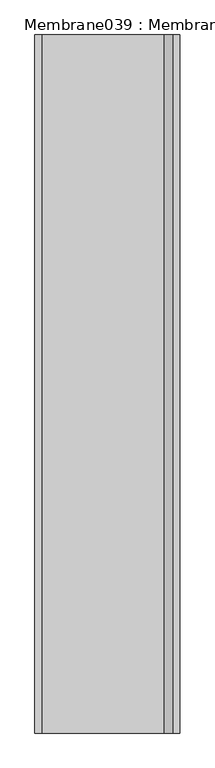
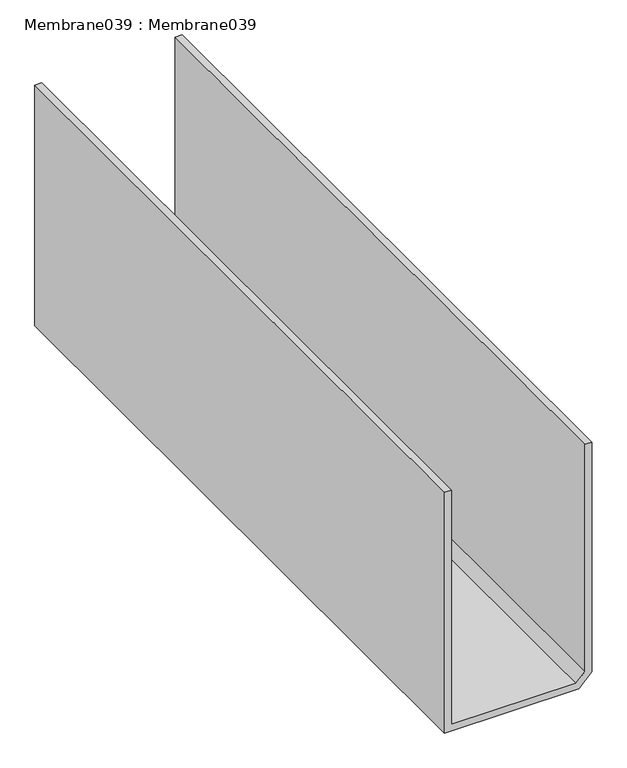
"""IFC4 building model written with IfcOpenShell, lengths in millimetres: proxy geometry, Membrane039 : Membrane039."""

from ifc_helpers import new_model, si_unit, frame, origin, place, context, project, spatial, polyline, outline, extrude, source, transform, mapped, element, save


def membrane039_membrane039_2a3038c1(model_context):
    return source(origin(), model_context, "Body", "SweptSolid", [
        extrude(outline(polyline([(33313.1445312, -9688.7902344), (32637.1367048, -9688.7902344), (32611.440625, -9714.2056282), (32611.440625, -10065.5505859), (33309.0146212, -10065.5505859), (33309.0146212, -10084.6005859), (32592.390625, -10084.6005859), (32592.390625, -9706.2535079), (32629.3071489, -9669.7402344), (33313.1445312, -9669.7402344), (33313.1445312, -9688.7902344)])), frame((0.0, 7982.1531721, 0.0), z_axis=(0.0, 1.0, 0.0), x_axis=(0.0, 0.0, 1.0)), (0.0, 0.0, 1.0), 2000.0),
    ])


if __name__ == "__main__":
    model = new_model("IFC4")
    model_context = context("Model", 3, world=origin())
    ifc_project = project(units=[si_unit("LENGTHUNIT", "METRE", prefix="MILLI")], contexts=[model_context])
    site = spatial("IfcSite", under=ifc_project)
    building = spatial("IfcBuilding", under=site)
    placement = place(None, origin())
    membrane039_membrane039_shape = membrane039_membrane039_2a3038c1(model_context)
    element("IfcBuildingElementProxy", 1, Name="Membrane039 : Membrane039", ObjectType="Membrane039 : Membrane039", at=placement, inside=building, context=model_context, shape_type="MappedRepresentation", body=[
        mapped(membrane039_membrane039_shape, transform((0.0, 0.0, 0.0), x_axis=(1.0, 0.0, 0.0), y_axis=(0.0, 1.0, 0.0), z_axis=(0.0, 0.0, 1.0))),
    ])
    save(model, "model.ifc")

# Revit data of these elements
# Type "Membrane039 : Membrane039"
#   NameOverride = "Membrane039"
# Element 1 (IfcBuildingElementProxy, "Membrane039 : Membrane039")
#   Materials on its faces: "3/4\" DRAINAGE CELL"
# Materials
#   "3/4\" DRAINAGE CELL": class "Unassigned", colour RGB 218 235 221, transparency 0, Cost = 0
